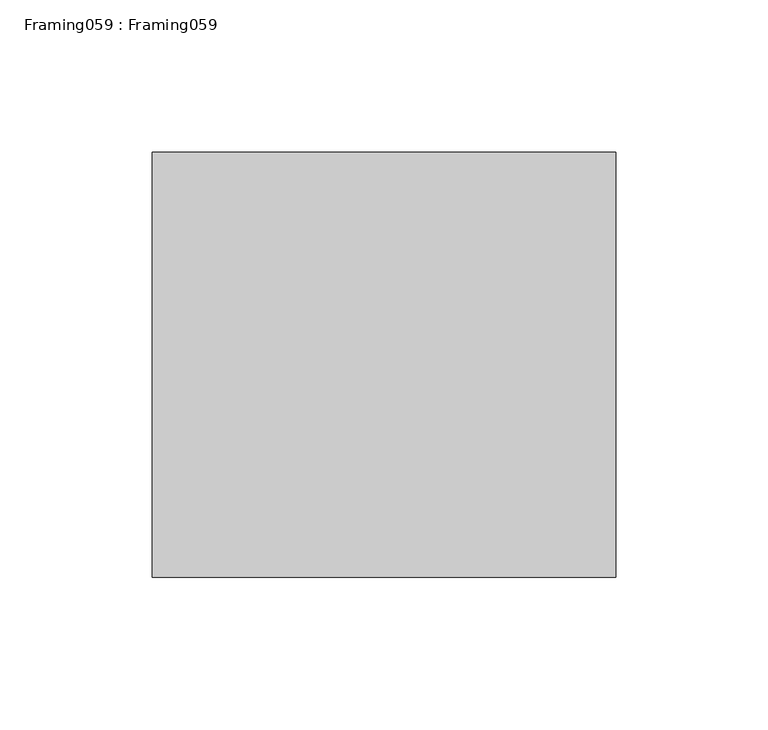
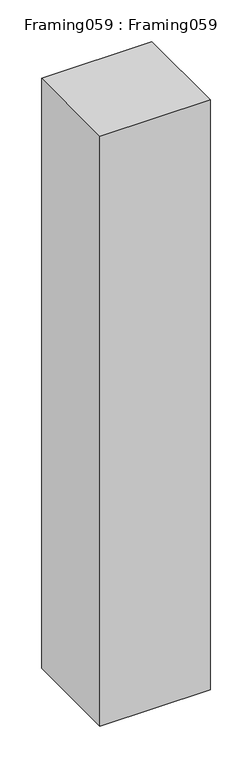
"""IFC4 building model written with IfcOpenShell, lengths in millimetres: proxy geometry, Framing059 : Framing059."""

from ifc_helpers import new_model, si_unit, frame, origin, place, context, project, spatial, polyline, outline, extrude, source, transform, mapped, element, save


def framing059_framing059_ee88b436(model_context):
    return source(origin(), model_context, "Body", "SweptSolid", [
        extrude(outline(polyline([(5694.2880859, 9730.3383229), (5694.2880859, 9590.6375834), (5541.8880859, 9590.6375834), (5541.8880859, 9730.3383229), (5694.2880859, 9730.3383229)])), frame((0.0, 0.0, 36582.096), z_axis=(0.0, 0.0, 1.0), x_axis=(1.0, 0.0, 0.0)), (0.0, 0.0, 1.0), 863.6),
    ])


if __name__ == "__main__":
    model = new_model("IFC4")
    model_context = context("Model", 3, world=origin())
    ifc_project = project(units=[si_unit("LENGTHUNIT", "METRE", prefix="MILLI")], contexts=[model_context])
    site = spatial("IfcSite", under=ifc_project)
    building = spatial("IfcBuilding", under=site)
    placement = place(None, origin())
    framing059_framing059_shape = framing059_framing059_ee88b436(model_context)
    element("IfcBuildingElementProxy", 1, Name="Framing059 : Framing059", ObjectType="Framing059 : Framing059", at=placement, inside=building, context=model_context, shape_type="MappedRepresentation", body=[
        mapped(framing059_framing059_shape, transform((0.0, 0.0, 0.0), x_axis=(1.0, 0.0, 0.0), y_axis=(0.0, 1.0, 0.0), z_axis=(0.0, 0.0, 1.0))),
    ])
    save(model, "model.ifc")

# Revit data of these elements
# Type "Framing059 : Framing059"
#   NameOverride = "Framing059"
# Element 1 (IfcBuildingElementProxy, "Framing059 : Framing059")
#   Materials on its faces: "WOOD FRAMING (SEE STRUCT DWGS)"
# Materials
#   "WOOD FRAMING (SEE STRUCT DWGS)": class "Unassigned", colour RGB 224 188 168, transparency 0, Cost = 0
